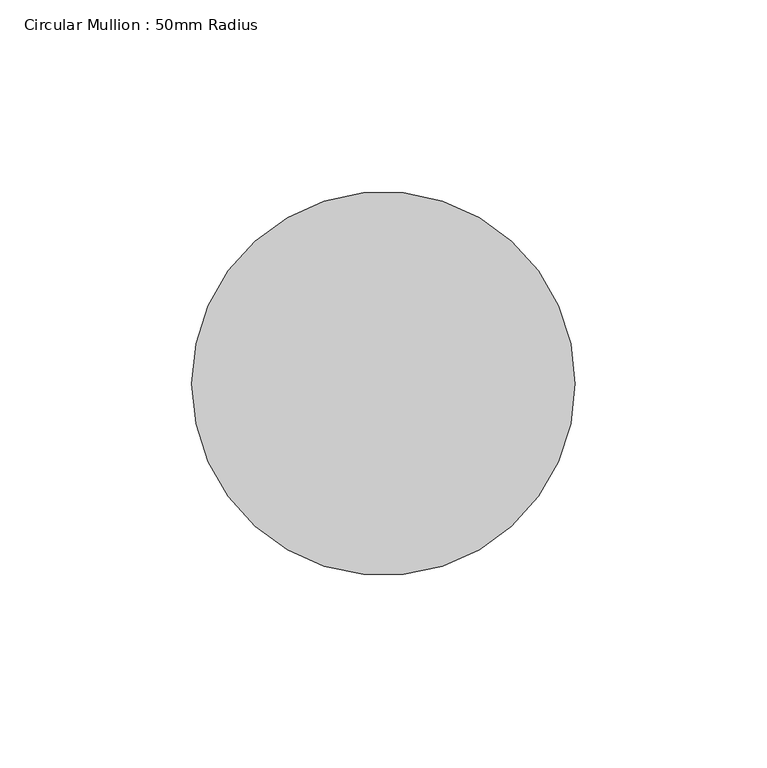
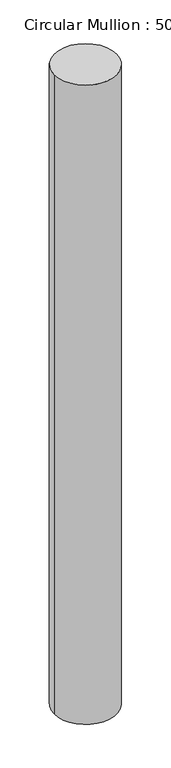
"""IFC4 building model written with IfcOpenShell, lengths in millimetres: member geometry, Circular Mullion : 50mm Radius."""

from ifc_helpers import new_model, si_unit, point, frame, origin, origin_2d, place, context, project, spatial, circle_curve, trimmed, segment, composite_curve, outline, extrude, source, transform, mapped, element, save


def circular_mullion_50mm_radius_7ca60f9b(model_context):
    return source(origin(), model_context, "Body", "SweptSolid", [
        extrude(outline(composite_curve([segment(trimmed(circle_curve(origin_2d(), 50.0), [point((50.0, 0.0))], [point((-50.0, 0.0))], False, "CARTESIAN"), True, "CONTINUOUS"), segment(trimmed(circle_curve(origin_2d(), 50.0), [point((-50.0, 0.0))], [point((50.0, 0.0))], False, "CARTESIAN"), True, "CONTINUOUS")], self_intersect=False)), frame((0.0, 0.0, -1080.3605914), z_axis=(0.0, 0.0, 1.0), x_axis=(1.0, 0.0, 0.0)), (0.0, 0.0, 1.0), 1080.3605914),
    ])


if __name__ == "__main__":
    model = new_model("IFC4")
    model_context = context("Model", 3, world=origin())
    ifc_project = project(units=[si_unit("LENGTHUNIT", "METRE", prefix="MILLI")], contexts=[model_context])
    site = spatial("IfcSite", under=ifc_project)
    building = spatial("IfcBuilding", under=site)
    placement = place(None, origin())
    circular_mullion_50mm_radius_shape = circular_mullion_50mm_radius_7ca60f9b(model_context)
    element("IfcMember", 1, ObjectType="Circular Mullion : 50mm Radius", at=placement, inside=building, context=model_context, shape_type="MappedRepresentation", body=[
        mapped(circular_mullion_50mm_radius_shape, transform((0.0, 0.0, 0.0), x_axis=(1.0, 0.0, 0.0), y_axis=(0.0, 1.0, 0.0), z_axis=(0.0, 0.0, 1.0))),
    ])
    save(model, "model.ifc")

# Revit data of these elements
# Type "Circular Mullion : 50mm Radius"
#   built-in parameter 1007350 = 0.164042 (stored number, unit not read)
# Element 1 (IfcMember, "Circular Mullion : 50mm Radius")
#   Materials on its faces: "Aluminium"
# Materials
#   "Aluminium": class "Metal", colour RGB 247 247 247, transparency 0, Description = "Aluminium 6061", Cost = 0
